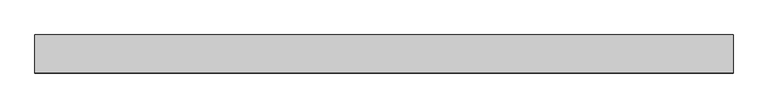
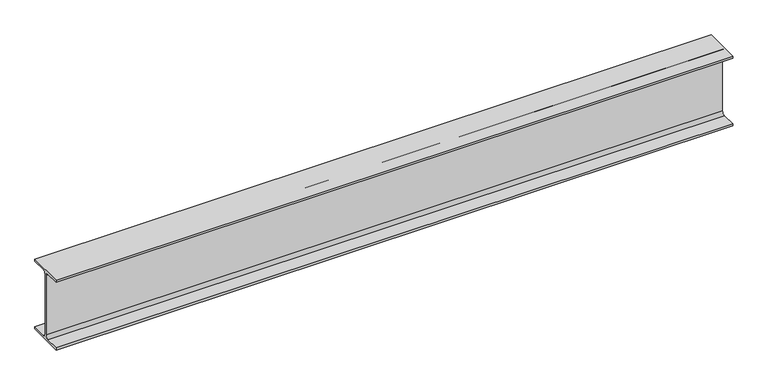
"""IFC4 building model written with IfcOpenShell, lengths in millimetres: beam geometry, Steel Framing_H_KS : H_SB_AR_S02_H-300x150x6.5x9_WG1."""

from ifc_helpers import new_model, si_unit, point, frame, frame_2d, origin, place, context, project, spatial, polyline, circle_curve, trimmed, segment, composite_curve, outline, extrude, source, transform, mapped, element, save


def beam_9f34c004(model_context):
    return source(origin(), model_context, "Body", "SweptSolid", [
        extrude(outline(composite_curve([segment(polyline([(75.0, -141.0), (75.0, -150.0), (-75.0, -150.0), (-75.0, -141.0), (-16.25, -141.0)]), True, "CONTINUOUS"), segment(trimmed(circle_curve(frame_2d((-16.25, -128.0)), 13.0), [point((-16.25, -141.0))], [point((-3.25, -128.0))], True, "CARTESIAN"), True, "CONTINUOUS"), segment(polyline([(-3.25, -128.0), (-3.25, 128.0)]), True, "CONTINUOUS"), segment(trimmed(circle_curve(frame_2d((-16.25, 128.0)), 13.0), [point((-3.25, 128.0))], [point((-16.25, 141.0))], True, "CARTESIAN"), True, "CONTINUOUS"), segment(polyline([(-16.25, 141.0), (-75.0, 141.0), (-75.0, 150.0), (75.0, 150.0), (75.0, 141.0), (16.25, 141.0)]), True, "CONTINUOUS"), segment(trimmed(circle_curve(frame_2d((16.25, 128.0)), 13.0), [point((16.25, 141.0))], [point((3.25, 128.0))], True, "CARTESIAN"), True, "CONTINUOUS"), segment(polyline([(3.25, 128.0), (3.25, -128.0)]), True, "CONTINUOUS"), segment(trimmed(circle_curve(frame_2d((16.25, -128.0)), 13.0), [point((3.25, -128.0))], [point((16.25, -141.0))], True, "CARTESIAN"), True, "CONTINUOUS"), segment(polyline([(16.25, -141.0), (75.0, -141.0)]), True, "CONTINUOUS")], self_intersect=False)), frame((-1412.3, 0.0, 0.0), z_axis=(1.0, 0.0, 0.0), x_axis=(0.0, 1.0, 0.0)), (0.0, 0.0, 1.0), 2749.6),
    ])


if __name__ == "__main__":
    model = new_model("IFC4")
    model_context = context("Model", 3, world=origin())
    ifc_project = project(units=[si_unit("LENGTHUNIT", "METRE", prefix="MILLI")], contexts=[model_context])
    site = spatial("IfcSite", under=ifc_project)
    building = spatial("IfcBuilding", under=site)
    placement = place(None, origin())
    beam_shape = beam_9f34c004(model_context)
    element("IfcBeam", 1, ObjectType="Steel Framing_H_KS : H_SB_AR_S02_H-300x150x6.5x9_WG1", at=placement, inside=building, context=model_context, shape_type="MappedRepresentation", body=[
        mapped(beam_shape, transform((0.0, 0.0, 0.0), x_axis=(1.0, 0.0, 0.0), y_axis=(0.0, 1.0, 0.0), z_axis=(0.0, 0.0, 1.0))),
    ])
    save(model, "model.ifc")

# Revit data of these elements
# Type "Steel Framing_H_KS : H_SB_AR_S02_H-300x150x6.5x9_WG1"
#   Type Comments = "MAIN"
#   Type Mark = "WG1"
#   H_SectionID = "H-300x150x6.5x9"
#   H_Ratio for Additional Steel Plate = 0.2
#   Width = 15.0 cm
#   Web Thickness = 0.65 cm
#   Web Fillet = 1.3 cm
#   Warping Constant = 107000.0 cm⁶
#   Torsional Moment of Inertia = 9.9539 cm⁴
#   Section Area = 46.78 cm²
#   Plastic Modulus weak axis = 105.0 cm³
#   Plastic Modulus strong axis = 542.0 cm³
#   Perimeter = 1.17 m²/m
#   Nominal Weight = 36.70 kgf/m
#   Moment of Inertia weak axis = 508.00 cm⁴
#   Moment of Inertia strong axis = 7210.00 cm⁴
#   Height = 30.0 cm
#   Flange Thickness = 0.9 cm
#   Elastic Modulus weak axis = 67.7 cm³
#   Elastic Modulus strong axis = 481.0 cm³
#   Centroid Vertical = 15.0 cm
#   Centroid Horizontal = 7.5 cm
#   Bolt Spacing = 8.89 cm
#   Length [instance default] = 1500 mm
#   Structural Material [instance default] = Steel, 45-345
#   Section Name Key = ""
#   Assembly Code = ""
# Element 1 (IfcBeam, "Steel Framing_H_KS : H_SB_AR_S02_H-300x150x6.5x9_WG1")
#   Materials on its faces: "Steel, 45-345"
# Materials
#   "Steel, 45-345": class "Metal", colour RGB 189 187 185, transparency 0, Description = "Steel 345 MPa", Cost = 0
